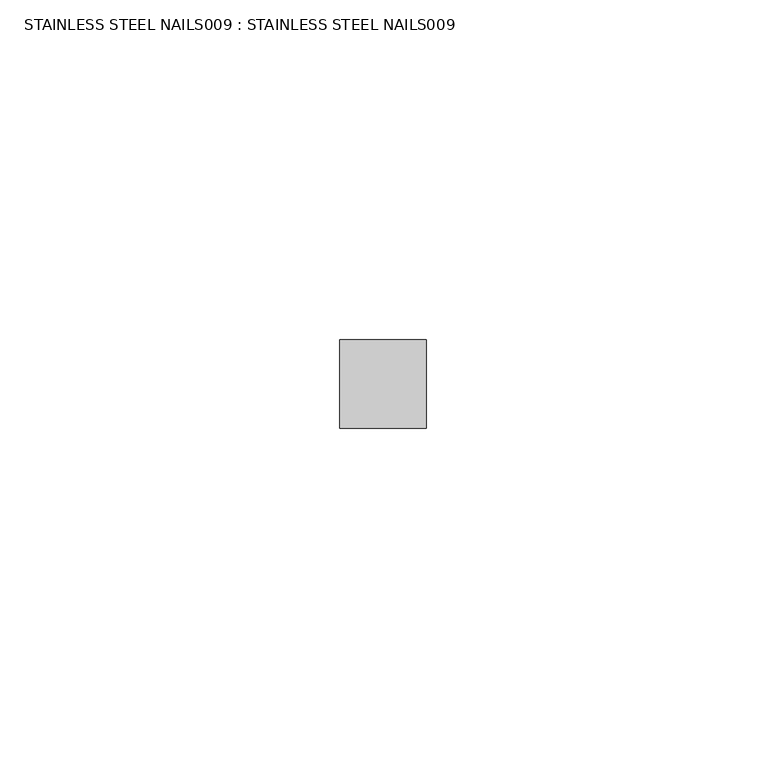
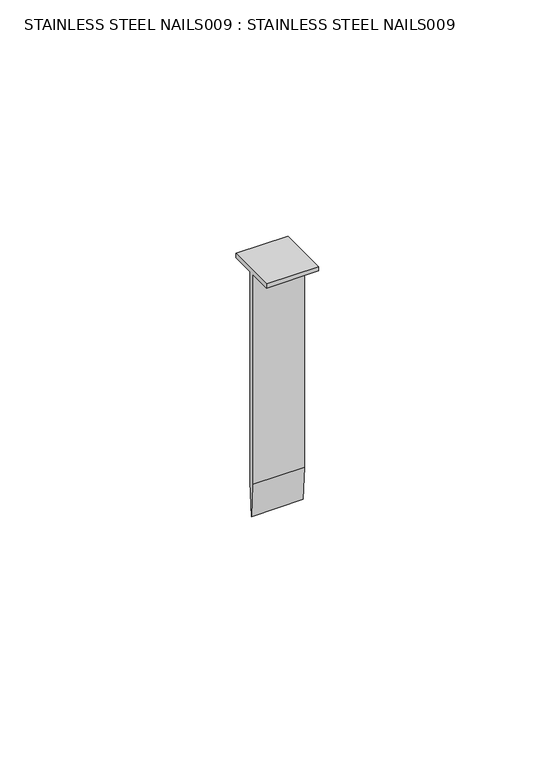
"""IFC4 building model written with IfcOpenShell, lengths in millimetres: proxy geometry, STAINLESS STEEL NAILS009 : STAINLESS STEEL NAILS009."""

from ifc_helpers import new_model, si_unit, frame, origin, place, context, project, spatial, polyline, outline, extrude, source, transform, mapped, element, save


def stainless_steel_nails009_stainless_steel_nails009_c75e95d3(model_context):
    return source(origin(), model_context, "Body", "SweptSolid", [
        extrude(outline(polyline([(-5490.4870231, 40241.4271837), (-5490.4870231, 40242.5103824), (-5477.4886393, 40242.5103824), (-5477.4886393, 40241.4271837), (-5483.4462319, 40241.4271837), (-5483.4462319, 40187.1010401), (-5483.9878312, 40178.4354508), (-5484.5294305, 40187.1010401), (-5484.5294305, 40241.4271837), (-5490.4870231, 40241.4271837)])), frame((14383.0178845, 0.0, 0.0), z_axis=(1.0, 0.0, 0.0), x_axis=(0.0, 1.0, 0.0)), (0.0, 0.0, 1.0), 12.7),
    ])


if __name__ == "__main__":
    model = new_model("IFC4")
    model_context = context("Model", 3, world=origin())
    ifc_project = project(units=[si_unit("LENGTHUNIT", "METRE", prefix="MILLI")], contexts=[model_context])
    site = spatial("IfcSite", under=ifc_project)
    building = spatial("IfcBuilding", under=site)
    placement = place(None, origin())
    stainless_steel_nails009_stainless_steel_nails009_shape = stainless_steel_nails009_stainless_steel_nails009_c75e95d3(model_context)
    element("IfcBuildingElementProxy", 1, Name="STAINLESS STEEL NAILS009 : STAINLESS STEEL NAILS009", ObjectType="STAINLESS STEEL NAILS009 : STAINLESS STEEL NAILS009", at=placement, inside=building, context=model_context, shape_type="MappedRepresentation", body=[
        mapped(stainless_steel_nails009_stainless_steel_nails009_shape, transform((0.0, 0.0, 0.0), x_axis=(1.0, 0.0, 0.0), y_axis=(0.0, 1.0, 0.0), z_axis=(0.0, 0.0, 1.0))),
    ])
    save(model, "model.ifc")

# Revit data of these elements
# Type "STAINLESS STEEL NAILS009 : STAINLESS STEEL NAILS009"
#   NameOverride = "STAINLESS STEEL NAILS009"
# Element 1 (IfcBuildingElementProxy, "STAINLESS STEEL NAILS009 : STAINLESS STEEL NAILS009")
#   Materials on its faces: "1 3/4\" STAINLESS STEEL RINGSHANK 5D COMMON NAILS @ 4\" (101.6MM) O.C. FIRESTONE PROVIDED MAX., 1/2\" STAGGERED"
# Materials
#   "1 3/4\" STAINLESS STEEL RINGSHANK 5D COMMON NAILS @ 4\" (101.6MM) O.C. FIRESTONE PROVIDED MAX., 1/2\" STAGGERED": class "Unassigned", colour RGB 255 255 255, transparency 0
